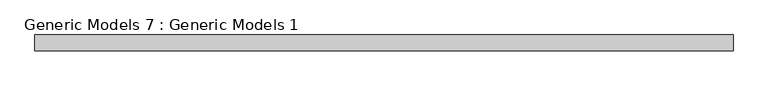
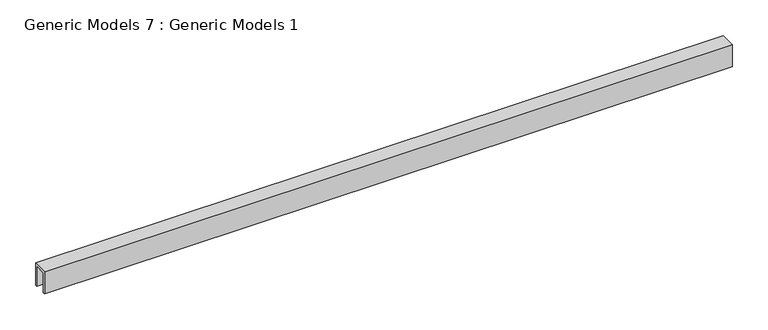
"""IFC4 building model written with IfcOpenShell, lengths in millimetres: proxy geometry, Generic Models 7 : Generic Models 1."""

from ifc_helpers import new_model, si_unit, frame, origin, place, context, project, spatial, polyline, outline, extrude, source, transform, mapped, element, save


def generic_models_7_generic_models_1_d984c418(model_context):
    return source(origin(), model_context, "Body", "SweptSolid", [
        extrude(outline(polyline([(39527.9428995, 2444.75), (39527.9428995, 2406.65), (39524.7678995, 2406.65), (39524.7678995, 2441.575), (39505.7178995, 2441.575), (39505.7178995, 2406.65), (39502.5428995, 2406.65), (39502.5428995, 2444.75), (39527.9428995, 2444.75)])), frame((51480.3077305, 0.0, 0.0), z_axis=(1.0, 0.0, 0.0), x_axis=(0.0, 1.0, 0.0)), (0.0, 0.0, 1.0), 1117.6),
    ])


if __name__ == "__main__":
    model = new_model("IFC4")
    model_context = context("Model", 3, world=origin())
    ifc_project = project(units=[si_unit("LENGTHUNIT", "METRE", prefix="MILLI")], contexts=[model_context])
    site = spatial("IfcSite", under=ifc_project)
    building = spatial("IfcBuilding", under=site)
    placement = place(None, origin())
    generic_models_7_generic_models_1_shape = generic_models_7_generic_models_1_d984c418(model_context)
    element("IfcBuildingElementProxy", 1, Name="Generic Models 7 : Generic Models 1", ObjectType="Generic Models 7 : Generic Models 1", at=placement, inside=building, context=model_context, shape_type="MappedRepresentation", body=[
        mapped(generic_models_7_generic_models_1_shape, transform((0.0, 0.0, 0.0), x_axis=(1.0, 0.0, 0.0), y_axis=(0.0, 1.0, 0.0), z_axis=(0.0, 0.0, 1.0))),
    ])
    save(model, "model.ifc")

# Revit data of these elements
# Element 1 (IfcBuildingElementProxy, "Generic Models 7 : Generic Models 1")
#   Materials on its faces: "ALUM. HEADER PROFILE TO MATCH EXISTING AT TENANT ENTRANCE"
# Materials
#   "ALUM. HEADER PROFILE TO MATCH EXISTING AT TENANT ENTRANCE": class "Unassigned", colour RGB 226 225 224, transparency 0, Cost = 0
